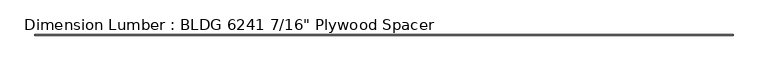
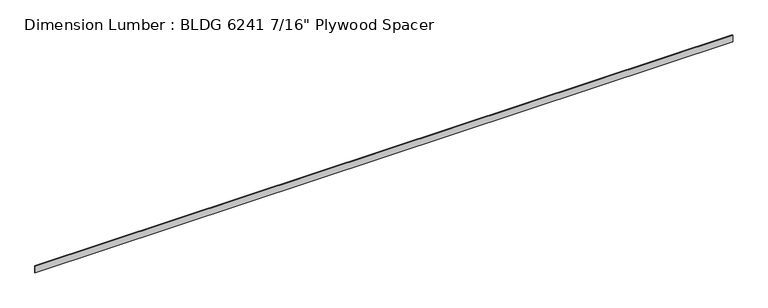
"""IFC4 building model written with IfcOpenShell, lengths in millimetres: beam geometry."""

from ifc_helpers import new_model, si_unit, frame, origin, place, context, project, spatial, polyline, outline, extrude, source, transform, mapped, element, save


def beam_af2566d3(model_context):
    return source(origin(), model_context, "Body", "SweptSolid", [
        extrude(outline(polyline([(6458.3020508, 5.55625), (6458.3020508, -5.55625), (-6159.1479492, -5.55625), (-6159.1479492, 5.55625), (6458.3020508, 5.55625)])), frame((0.0, 0.0, -63.5), z_axis=(0.0, 0.0, 1.0), x_axis=(1.0, 0.0, 0.0)), (0.0, 0.0, 1.0), 127.0),
    ])


if __name__ == "__main__":
    model = new_model("IFC4")
    model_context = context("Model", 3, world=origin())
    ifc_project = project(units=[si_unit("LENGTHUNIT", "METRE", prefix="MILLI")], contexts=[model_context])
    site = spatial("IfcSite", under=ifc_project)
    building = spatial("IfcBuilding", under=site)
    placement = place(None, origin())
    beam_shape = beam_af2566d3(model_context)
    element("IfcBeam", 1, ObjectType="Dimension Lumber : BLDG 6241 7/16\" Plywood Spacer", at=placement, inside=building, context=model_context, shape_type="MappedRepresentation", body=[
        mapped(beam_shape, transform((0.0, 0.0, 0.0), x_axis=(1.0, 0.0, 0.0), y_axis=(0.0, 1.0, 0.0), z_axis=(0.0, 0.0, 1.0))),
    ])
    save(model, "model.ifc")

# Revit data of these elements
# Type "Dimension Lumber : BLDG 6241 7/16\" Plywood Spacer"
#   Assembly Code = "B10"
#   A = 0.273472 SF
#   Length [instance default] = 5' - 0"
#   b = 0' - 0 7/16"
#   d = 0' - 5"
#   Structural Material [instance default] = Softwood, Lumber
# Element 1 (IfcBeam, "Dimension Lumber : BLDG 6241 7/16\" Plywood Spacer")
#   Structural Material = Plywood, Sheathing
#   Materials on its faces: "Plywood, Sheathing"
# Materials
#   "Softwood, Lumber": class "Wood", colour RGB 223 192 134, transparency 0, Description = "Pinus Echinata", Cost = 0
#   "Plywood, Sheathing": class "Wood", colour RGB 212 179 113, transparency 0, Description = "Plywood, sheathing grade", Cost = 0
